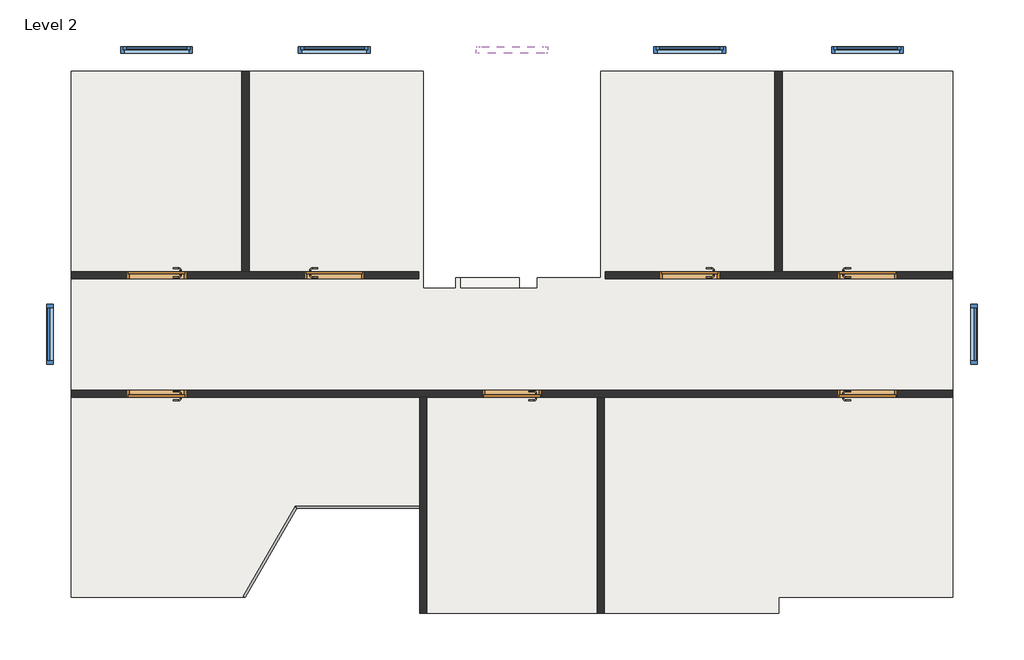
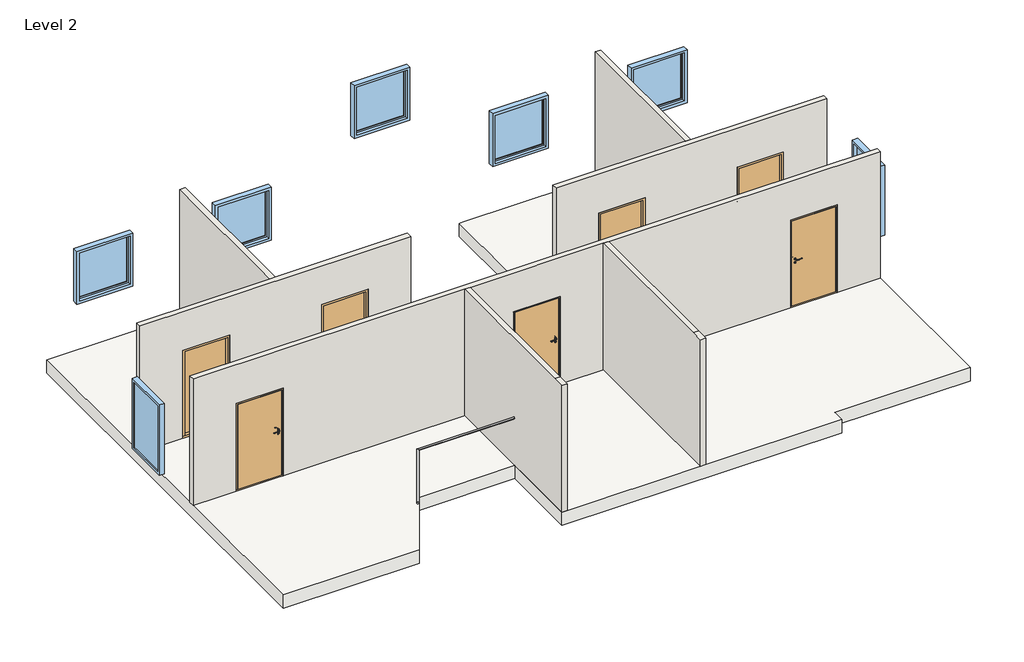
# One storey: 7 doors, 7 walls, 7 windows, 1 railing, 1 slab.
"""IFC4 building model written with IfcOpenShell, lengths in millimetres."""

import ifcopenshell
import ifcopenshell.guid

model = None  # the IFC model being written
_history = None  # IfcOwnerHistory: only IFC2X3 demands one
_inside = {}  # id of a spatial element -> (the spatial element, [elements in it])
_under = {}  # id of a project, library or spatial element -> (it, [spatial elements below it])
_declared = {}  # id of a project -> (the project, [libraries it declares])
_typed = {}  # id of a type object -> (the type object, [elements of that type])
_made_of = {}  # id of a material, layer set ... -> (it, [elements and type objects made of it])


def new_model(schema):
    """Start an empty IFC model of exactly this schema.

    Asked for "IFC4X3", IfcOpenShell would pick the latest addendum, in which some entities
    have other attributes; the version numbers below select the first issue.
    IFC2X3 requires an IfcOwnerHistory on every rooted entity: one is made here for all.
    """
    global model, _history
    if schema == "IFC4X3":
        model = ifcopenshell.file(schema_version=(4, 3, 0, 0))
    else:
        model = ifcopenshell.file(schema=schema)
    _inside.clear()
    _under.clear()
    _declared.clear()
    _typed.clear()
    _made_of.clear()
    _history = None
    if model.schema == "IFC2X3":
        org = make("IfcOrganization", Name="unknown")
        user = make(
            "IfcPersonAndOrganization",
            ThePerson=make("IfcPerson", FamilyName="unknown"),
            TheOrganization=org,
        )
        app = make(
            "IfcApplication",
            ApplicationDeveloper=org,
            Version="unknown",
            ApplicationFullName="unknown",
            ApplicationIdentifier="unknown",
        )
        _history = make(
            "IfcOwnerHistory",
            OwningUser=user,
            OwningApplication=app,
            ChangeAction="ADDED",
            CreationDate=0,
        )
    return model


def make(cls, **values):
    """One entity of the class cls with the attributes given. An attribute that is None is left unset."""
    return model.create_entity(
        cls, **{name: value for name, value in values.items() if value is not None}
    )


def rooted(cls, **values):
    """An entity with a GlobalId (a new one), such as an element, a storey or a relation."""
    return make(cls, GlobalId=ifcopenshell.guid.new(), OwnerHistory=_history, **values)


def si_unit(unit_type, name, prefix=None):
    """IfcSIUnit, for example si_unit("LENGTHUNIT", "METRE", prefix="MILLI")."""
    return make("IfcSIUnit", UnitType=unit_type, Prefix=prefix, Name=name)


def assignment(units):
    """IfcUnitAssignment: the units of a project."""
    return None if units is None else make("IfcUnitAssignment", Units=units)


def point(xyz):
    """IfcCartesianPoint."""
    return None if xyz is None else make("IfcCartesianPoint", Coordinates=xyz)


def direction(xyz):
    """IfcDirection."""
    return None if xyz is None else make("IfcDirection", DirectionRatios=xyz)


def frame(location, z_axis=None, x_axis=None):
    """IfcAxis2Placement3D, a coordinate frame: its origin and axes. An axis left out is left unset."""
    return make(
        "IfcAxis2Placement3D",
        Location=point(location),
        Axis=direction(z_axis),
        RefDirection=direction(x_axis),
    )


def frame_2d(location, x_axis=None):
    """IfcAxis2Placement2D, a coordinate frame in the plane: its origin and x axis."""
    return make(
        "IfcAxis2Placement2D", Location=point(location), RefDirection=direction(x_axis)
    )


def origin():
    """The frame at (0, 0, 0) with its axes left unset."""
    return frame((0.0, 0.0, 0.0))


def place(relative_to, where):
    """IfcLocalPlacement: puts the frame where relative to a parent placement (None: the world)."""
    return make(
        "IfcLocalPlacement", PlacementRelTo=relative_to, RelativePlacement=where
    )


def context(
    kind, dimensions, precision=None, world=None, true_north=None, identifier=None
):
    """IfcGeometricRepresentationContext, for example the 3D "Model" context."""
    return make(
        "IfcGeometricRepresentationContext",
        ContextIdentifier=identifier,
        ContextType=kind,
        CoordinateSpaceDimension=dimensions,
        Precision=precision,
        WorldCoordinateSystem=world,
        TrueNorth=true_north,
    )


def project(units=None, contexts=None):
    """IfcProject with its units and contexts."""
    return rooted(
        "IfcProject",
        Name="project",
        RepresentationContexts=contexts,
        UnitsInContext=assignment(units),
    )


def spatial(cls, under=None, at=None, **own):
    """A site, building, storey or space (cls), placed at a placement, below another one or the project."""
    s = rooted(cls, ObjectPlacement=at, **own)
    if under is not None:
        _under.setdefault(under.id(), (under, []))[1].append(s)
    return s


def polyline(points):
    """IfcPolyline through the points."""
    return make("IfcPolyline", Points=[point(p) for p in points])


def circle_curve(where, radius):
    """IfcCircle in the frame where."""
    return make("IfcCircle", Position=where, Radius=radius)


def ellipse_curve(where, semi_axis1, semi_axis2):
    """IfcEllipse in the frame where."""
    return make(
        "IfcEllipse", Position=where, SemiAxis1=semi_axis1, SemiAxis2=semi_axis2
    )


def trimmed(basis, trim1, trim2, sense, master):
    """IfcTrimmedCurve: the piece of a basis curve between two trims."""
    return make(
        "IfcTrimmedCurve",
        BasisCurve=basis,
        Trim1=trim1,
        Trim2=trim2,
        SenseAgreement=sense,
        MasterRepresentation=master,
    )


def segment(curve, same_sense, transition):
    """IfcCompositeCurveSegment."""
    return make(
        "IfcCompositeCurveSegment",
        Transition=transition,
        SameSense=same_sense,
        ParentCurve=curve,
    )


def composite_curve(segments, self_intersect=None):
    """IfcCompositeCurve: segments joined end to end."""
    return make("IfcCompositeCurve", Segments=segments, SelfIntersect=self_intersect)


def outline(outer, holes=None, kind="AREA"):
    """IfcArbitraryClosedProfileDef: a profile drawn as a closed curve; with holes, ...WithVoids."""
    if holes is None:
        return make("IfcArbitraryClosedProfileDef", ProfileType=kind, OuterCurve=outer)
    return make(
        "IfcArbitraryProfileDefWithVoids",
        ProfileType=kind,
        OuterCurve=outer,
        InnerCurves=holes,
    )


def extrude(swept, where, along, depth):
    """IfcExtrudedAreaSolid: the profile swept, set in the frame where, extruded along a direction by depth."""
    return make(
        "IfcExtrudedAreaSolid",
        SweptArea=swept,
        Position=where,
        ExtrudedDirection=direction(along),
        Depth=depth,
    )


def faces_of(points, faces, orient=None, outer=None):
    """IfcFace entities. A face is a list of loops; a loop is a list of indices into points, from 0.

    orient and outer hold one flag for each loop. By default every Orientation is true, the
    first loop of a face is its IfcFaceOuterBound and the others are IfcFaceBound.
    """
    made = []
    for i, loops in enumerate(faces):
        bounds = []
        for j, loop in enumerate(loops):
            is_outer = j == 0 if outer is None else outer[i][j]
            bounds.append(
                make(
                    "IfcFaceOuterBound" if is_outer else "IfcFaceBound",
                    Bound=make("IfcPolyLoop", Polygon=[points[k] for k in loop]),
                    Orientation=True if orient is None else orient[i][j],
                )
            )
        made.append(make("IfcFace", Bounds=bounds))
    return made


def faceted_brep(points, faces, orient=None, outer=None, voids=None):
    """IfcFacetedBrep: a solid bounded by flat faces; with voids (closed shells), ...WithVoids."""
    shared = [point(p) for p in points]
    hull = make("IfcClosedShell", CfsFaces=faces_of(shared, faces, orient, outer))
    if voids is None:
        return make("IfcFacetedBrep", Outer=hull)
    return make(
        "IfcFacetedBrepWithVoids",
        Outer=hull,
        Voids=[
            make(cls, CfsFaces=faces_of(shared, fs, o, b)) for cls, fs, o, b in voids
        ],
    )


def shape(context_of_items, identifier, shape_type, items):
    """IfcShapeRepresentation: the items that make up one representation, for example the "Body"."""
    return make(
        "IfcShapeRepresentation",
        ContextOfItems=context_of_items,
        RepresentationIdentifier=identifier,
        RepresentationType=shape_type,
        Items=items,
    )


def source(mapping_origin, context_of_items, identifier, shape_type, items):
    """IfcRepresentationMap: a shape defined once, which mapped items show again and again."""
    return make(
        "IfcRepresentationMap",
        MappingOrigin=mapping_origin,
        MappedRepresentation=shape(context_of_items, identifier, shape_type, items),
    )


def transform(
    local_origin,
    x_axis=None,
    y_axis=None,
    z_axis=None,
    scale=None,
    scale2=None,
    scale3=None,
    uniform=True,
):
    """IfcCartesianTransformationOperator3D, or its non-uniform kind. x_axis, y_axis, z_axis: its Axis1, 2, 3."""
    if uniform:
        return make(
            "IfcCartesianTransformationOperator3D",
            Axis1=direction(x_axis),
            Axis2=direction(y_axis),
            LocalOrigin=point(local_origin),
            Scale=scale,
            Axis3=direction(z_axis),
        )
    return make(
        "IfcCartesianTransformationOperator3DnonUniform",
        Axis1=direction(x_axis),
        Axis2=direction(y_axis),
        LocalOrigin=point(local_origin),
        Scale=scale,
        Axis3=direction(z_axis),
        Scale2=scale2,
        Scale3=scale3,
    )


def mapped(mapping_source, mapping_target):
    """IfcMappedItem: shows the shape of a source again, moved by a transform."""
    return make(
        "IfcMappedItem", MappingSource=mapping_source, MappingTarget=mapping_target
    )


def made_of(thing, what):
    """Note that an element or type object is made of a material, layer set ...; save() writes the relation."""
    if what is not None:
        _made_of.setdefault(what.id(), (what, []))[1].append(thing)
    return thing


def element(
    cls,
    number,
    at=None,
    inside=None,
    cuts=None,
    type_object=None,
    material=None,
    context=None,
    identifier="Body",
    shape_type=None,
    held_by="IfcProductDefinitionShape",
    body=None,
    shapes=None,
    **own,
):
    """One element of the class cls, such as IfcWall. Its Tag is "e" and its number.

    at: its placement. inside: the storey or other place that contains it. cuts: it is an
    opening in that element (IfcRelVoidsElement). A single representation is given by context,
    identifier, shape_type and body (its items); several are given by shapes. held_by: the class
    of the entity that holds the representations. save() writes the other relations.
    """
    e = rooted(cls, Tag="e%d" % number, ObjectPlacement=at, **own)
    if body is not None:
        shapes = [shape(context, identifier, shape_type, body)]
    if shapes is not None:
        e.Representation = make(held_by, Representations=shapes)
    if inside is not None:
        _inside.setdefault(inside.id(), (inside, []))[1].append(e)
    if cuts is not None:
        rooted(
            "IfcRelVoidsElement", RelatingBuildingElement=cuts, RelatedOpeningElement=e
        )
    if type_object is not None:
        _typed.setdefault(type_object.id(), (type_object, []))[1].append(e)
    return made_of(e, material)


def aggregate(whole, parts):
    """IfcRelAggregates: a whole, such as a stair, and the parts it consists of."""
    return rooted("IfcRelAggregates", RelatingObject=whole, RelatedObjects=parts)


def save(model, path):
    """Write the relations noted so far, then the file.

    IfcRelAggregates (storeys below a building ...), IfcRelContainedInSpatialStructure (elements
    in a storey), IfcRelDefinesByType, IfcRelAssociatesMaterial and IfcRelDeclares: one each for
    every whole, place, type object, material and project.
    """
    for whole, parts in _under.values():
        aggregate(whole, parts)
    for where, things in _inside.values():
        rooted(
            "IfcRelContainedInSpatialStructure",
            RelatedElements=things,
            RelatingStructure=where,
        )
    for kind, things in _typed.values():
        rooted("IfcRelDefinesByType", RelatedObjects=things, RelatingType=kind)
    for what, things in _made_of.values():
        rooted("IfcRelAssociatesMaterial", RelatedObjects=things, RelatingMaterial=what)
    for by, libraries in _declared.values():
        rooted("IfcRelDeclares", RelatingContext=by, RelatedDefinitions=libraries)
    model.write(path)


def plane_surface(at):
    """IfcPlane: the flat surface through the origin of the frame at, square to its z axis."""
    return make("IfcPlane", Position=at)


def cylinder_surface(at, radius):
    """IfcCylindricalSurface: all points at the distance radius from the z axis of the frame at."""
    return make("IfcCylindricalSurface", Position=at, Radius=radius)


def revolved_surface(curve, axis_point, axis_direction):
    """IfcSurfaceOfRevolution: the curve turned about the line through axis_point along axis_direction."""
    return make(
        "IfcSurfaceOfRevolution",
        SweptCurve=make("IfcArbitraryOpenProfileDef", ProfileType="CURVE", Curve=curve),
        AxisPosition=make("IfcAxis1Placement", Location=point(axis_point), Axis=direction(axis_direction)),
    )


def advanced_brep(points, edges, surfaces, faces):
    """IfcAdvancedBrep: a solid bounded by faces that lie on surfaces and meet in shared edges.

    An edge is (start, end): straight between two places in points (the first is 0);
    or (start, end, curve); or (start, end, curve, False) where it runs against its curve.
    A face is (place in surfaces, loops), or (place, loops, False) where it looks against
    its surface's normal. A loop lists edges by number (the first is 1), with a minus sign
    where the edge is run from its end to its start. The first loop is the outer one.
    """
    corners = [point(p) for p in points]
    vertices = [make("IfcVertexPoint", VertexGeometry=c) for c in corners]
    made = []
    for start, end, *more in edges:
        made.append(
            make(
                "IfcEdgeCurve",
                EdgeStart=vertices[start],
                EdgeEnd=vertices[end],
                EdgeGeometry=more[0] if more else make("IfcPolyline", Points=[corners[start], corners[end]]),
                SameSense=more[1] if len(more) > 1 else True,
            )
        )
    hull = []
    for where, loops, *sense in faces:
        bounds = []
        for j, loop in enumerate(loops):
            ring = [make("IfcOrientedEdge", EdgeElement=made[abs(k) - 1], Orientation=k > 0) for k in loop]
            bounds.append(
                make(
                    "IfcFaceOuterBound" if j == 0 else "IfcFaceBound",
                    Bound=make("IfcEdgeLoop", EdgeList=ring),
                    Orientation=True,
                )
            )
        hull.append(make("IfcAdvancedFace", Bounds=bounds, FaceSurface=surfaces[where], SameSense=sense[0] if sense else True))
    return make("IfcAdvancedBrep", Outer=make("IfcClosedShell", CfsFaces=hull))


def int_single_flush_10x20m_e84bf50b(model_context):
    return source(origin(), model_context, "Body", "SolidModel", [
        extrude(outline(composite_curve([segment(trimmed(circle_curve(frame_2d((1090.0, -406.0)), 20.0), [point((1070.0, -406.0))], [point((1110.0, -406.0))], False, "CARTESIAN"), True, "CONTINUOUS"), segment(trimmed(circle_curve(frame_2d((1090.0, -406.0)), 20.0), [point((1110.0, -406.0))], [point((1070.0, -406.0))], False, "CARTESIAN"), True, "CONTINUOUS")], self_intersect=False)), frame((0.0, 60.0, 0.0), z_axis=(0.0, 1.0, 0.0), x_axis=(0.0, 0.0, 1.0)), (0.0, 0.0, 1.0), 2.0),
        advanced_brep(
        [(-413.5, 62.0, 1090.0), (-398.5, 62.0, 1090.0), (-413.5, 84.5, 1090.0), (-398.5, 84.5, 1090.0), (-376.0, 107.0, 1090.0), (-376.0, 122.0, 1090.0), (-281.0, 122.0, 1090.0), (-281.0, 107.0, 1090.0)],
        [
            (0, 1, circle_curve(frame((-406.0, 62.0, 1090.0), z_axis=(0.0, -1.0, 0.0), x_axis=(1.0, 0.0, 0.0)), 7.5)),
            (1, 0, circle_curve(frame((-406.0, 62.0, 1090.0), z_axis=(0.0, -1.0, 0.0), x_axis=(1.0, 0.0, 0.0)), 7.5)),
            (0, 2),
            (2, 3, circle_curve(frame((-406.0, 84.5, 1090.0), z_axis=(0.0, -1.0, 0.0), x_axis=(1.0, 0.0, 0.0)), 7.5)),
            (3, 1),
            (3, 2, circle_curve(frame((-406.0, 84.5, 1090.0), z_axis=(0.0, -1.0, 0.0), x_axis=(1.0, 0.0, 0.0)), 7.5)),
            (4, 3, circle_curve(frame((-376.0, 84.5, 1090.0), z_axis=(0.0, 0.0, 1.0), x_axis=(-1.0, 0.0, 0.0)), 22.5)),
            (2, 5, circle_curve(frame((-376.0, 84.5, 1090.0), z_axis=(0.0, 0.0, -1.0), x_axis=(-1.0, 0.0, 0.0)), 37.5)),
            (5, 4, circle_curve(frame((-376.0, 114.5, 1090.0), z_axis=(-1.0, 0.0, 0.0), x_axis=(0.0, -1.0, 0.0)), 7.5)),
            (4, 5, circle_curve(frame((-376.0, 114.5, 1090.0), z_axis=(-1.0, 0.0, 0.0), x_axis=(0.0, -1.0, 0.0)), 7.5)),
            (5, 6),
            (6, 7, circle_curve(frame((-281.0, 114.5, 1090.0), z_axis=(-1.0, 0.0, 0.0), x_axis=(0.0, -1.0, 0.0)), 7.5)),
            (7, 4),
            (7, 6, circle_curve(frame((-281.0, 114.5, 1090.0), z_axis=(-1.0, 0.0, 0.0), x_axis=(0.0, -1.0, 0.0)), 7.5)),
        ],
        [
            plane_surface(frame((-406.0, 62.0, 1090.0), z_axis=(0.0, -1.0, 0.0), x_axis=(0.0, 0.0, -1.0))),
            cylinder_surface(frame((-406.0, 62.0, 1090.0), z_axis=(0.0, -1.0, 0.0), x_axis=(1.0, 0.0, 0.0)), 7.5),
            revolved_surface(trimmed(ellipse_curve(frame((-406.0, 84.5, 1090.0), z_axis=(0.0, -1.0, 0.0), x_axis=(1.0, 0.0, 0.0)), 7.5, 7.5), [point((-413.5, 84.5, 1090.0))], [point((-398.5, 84.5, 1090.0))], True, "CARTESIAN"), (-376.0, 84.5, 1090.0), (0.0, 0.0, -1.0)),
            revolved_surface(trimmed(ellipse_curve(frame((-406.0, 84.5, 1090.0), z_axis=(0.0, -1.0, 0.0), x_axis=(1.0, 0.0, 0.0)), 7.5, 7.5), [point((-398.5, 84.5, 1090.0))], [point((-413.5, 84.5, 1090.0))], True, "CARTESIAN"), (-376.0, 84.5, 1090.0), (0.0, 0.0, -1.0)),
            cylinder_surface(frame((-376.0, 114.5, 1090.0), z_axis=(-1.0, 0.0, 0.0), x_axis=(0.0, -1.0, 0.0)), 7.5),
            plane_surface(frame((-281.0, 114.5, 1090.0), z_axis=(1.0, 0.0, 0.0), x_axis=(0.0, 0.0, -1.0))),
        ],
        [
            (0, [[1, 2]]),
            (1, [[-1, 3, 4, 5]]),
            (1, [[-2, -5, 6, -3]]),
            (2, [[7, -4, 8, 9]]),
            (3, [[-8, -6, -7, 10]]),
            (4, [[-9, 11, 12, 13]]),
            (4, [[-10, -13, 14, -11]]),
            (5, [[-14, -12]]),
        ],
    ),
        extrude(outline(composite_curve([segment(trimmed(circle_curve(frame_2d((1010.0, -406.0)), 20.0), [point((990.0, -406.0))], [point((1030.0, -406.0))], False, "CARTESIAN"), True, "CONTINUOUS"), segment(trimmed(circle_curve(frame_2d((1010.0, -406.0)), 20.0), [point((1030.0, -406.0))], [point((990.0, -406.0))], False, "CARTESIAN"), True, "CONTINUOUS")], self_intersect=False), holes=[composite_curve([segment(trimmed(circle_curve(frame_2d((1015.0, -406.0)), 3.0), [point((1012.4019238, -407.5))], [point((1012.4019238, -404.5))], True, "CARTESIAN"), True, "CONTINUOUS"), segment(polyline([(1012.4019238, -404.5), (1000.0, -404.5), (1000.0, -407.5), (1012.4019238, -407.5)]), True, "CONTINUOUS")], self_intersect=False)]), frame((0.0, 60.0, 0.0), z_axis=(0.0, 1.0, 0.0), x_axis=(0.0, 0.0, 1.0)), (0.0, 0.0, 1.0), 2.0),
        extrude(outline(composite_curve([segment(trimmed(circle_curve(frame_2d((1090.0, -406.0)), 20.0), [point((1070.0, -406.0))], [point((1110.0, -406.0))], False, "CARTESIAN"), True, "CONTINUOUS"), segment(trimmed(circle_curve(frame_2d((1090.0, -406.0)), 20.0), [point((1110.0, -406.0))], [point((1070.0, -406.0))], False, "CARTESIAN"), True, "CONTINUOUS")], self_intersect=False)), frame((0.0, 18.0, 0.0), z_axis=(0.0, 1.0, 0.0), x_axis=(0.0, 0.0, 1.0)), (0.0, 0.0, 1.0), 2.0),
        advanced_brep(
        [(-413.5, 18.0, 1090.0), (-398.5, 18.0, 1090.0), (-398.5, -4.5, 1090.0), (-413.5, -4.5, 1090.0), (-376.0, -27.0, 1090.0), (-376.0, -42.0, 1090.0), (-281.0, -27.0, 1090.0), (-281.0, -42.0, 1090.0)],
        [
            (0, 1, circle_curve(frame((-406.0, 18.0, 1090.0), z_axis=(0.0, 1.0, 0.0), x_axis=(1.0, 0.0, 0.0)), 7.5)),
            (1, 0, circle_curve(frame((-406.0, 18.0, 1090.0), z_axis=(0.0, 1.0, 0.0), x_axis=(1.0, 0.0, 0.0)), 7.5)),
            (1, 2),
            (2, 3, circle_curve(frame((-406.0, -4.5, 1090.0), z_axis=(0.0, 1.0, 0.0), x_axis=(1.0, 0.0, 0.0)), 7.5)),
            (3, 0),
            (3, 2, circle_curve(frame((-406.0, -4.5, 1090.0), z_axis=(0.0, 1.0, 0.0), x_axis=(1.0, 0.0, 0.0)), 7.5)),
            (4, 5, circle_curve(frame((-376.0, -34.5, 1090.0), z_axis=(-1.0, 0.0, 0.0), x_axis=(0.0, 1.0, 0.0)), 7.5)),
            (5, 3, circle_curve(frame((-376.0, -4.5, 1090.0), z_axis=(0.0, 0.0, -1.0), x_axis=(-1.0, 0.0, 0.0)), 37.5)),
            (2, 4, circle_curve(frame((-376.0, -4.5, 1090.0), z_axis=(0.0, 0.0, 1.0), x_axis=(-1.0, 0.0, 0.0)), 22.5)),
            (5, 4, circle_curve(frame((-376.0, -34.5, 1090.0), z_axis=(-1.0, 0.0, 0.0), x_axis=(0.0, 1.0, 0.0)), 7.5)),
            (4, 6),
            (6, 7, circle_curve(frame((-281.0, -34.5, 1090.0), z_axis=(-1.0, 0.0, 0.0), x_axis=(0.0, 1.0, 0.0)), 7.5)),
            (7, 5),
            (7, 6, circle_curve(frame((-281.0, -34.5, 1090.0), z_axis=(-1.0, 0.0, 0.0), x_axis=(0.0, 1.0, 0.0)), 7.5)),
        ],
        [
            plane_surface(frame((-406.0, 18.0, 1090.0), z_axis=(0.0, 1.0, 0.0), x_axis=(0.0, 0.0, -1.0))),
            cylinder_surface(frame((-406.0, 18.0, 1090.0), z_axis=(0.0, 1.0, 0.0), x_axis=(1.0, 0.0, 0.0)), 7.5),
            revolved_surface(trimmed(ellipse_curve(frame((-406.0, -4.5, 1090.0), z_axis=(0.0, -1.0, 0.0), x_axis=(1.0, 0.0, 0.0)), 7.5, 7.5), [point((-413.5, -4.5, 1090.0))], [point((-398.5, -4.5, 1090.0))], True, "CARTESIAN"), (-376.0, -4.5, 1090.0), (0.0, 0.0, -1.0)),
            revolved_surface(trimmed(ellipse_curve(frame((-406.0, -4.5, 1090.0), z_axis=(0.0, -1.0, 0.0), x_axis=(1.0, 0.0, 0.0)), 7.5, 7.5), [point((-398.5, -4.5, 1090.0))], [point((-413.5, -4.5, 1090.0))], True, "CARTESIAN"), (-376.0, -4.5, 1090.0), (0.0, 0.0, -1.0)),
            cylinder_surface(frame((-376.0, -34.5, 1090.0), z_axis=(-1.0, 0.0, 0.0), x_axis=(0.0, 1.0, 0.0)), 7.5),
            plane_surface(frame((-281.0, -34.5, 1090.0), z_axis=(1.0, 0.0, 0.0), x_axis=(0.0, 0.0, -1.0))),
        ],
        [
            (0, [[1, 2]]),
            (1, [[3, 4, 5, -2]]),
            (1, [[-5, 6, -3, -1]]),
            (2, [[7, 8, -4, 9]]),
            (3, [[10, -9, -6, -8]]),
            (4, [[11, 12, 13, -7]]),
            (4, [[-13, 14, -11, -10]]),
            (5, [[-12, -14]]),
        ],
    ),
        extrude(outline(composite_curve([segment(trimmed(circle_curve(frame_2d((1010.0, -406.0)), 20.0), [point((990.0, -406.0))], [point((1030.0, -406.0))], False, "CARTESIAN"), True, "CONTINUOUS"), segment(trimmed(circle_curve(frame_2d((1010.0, -406.0)), 20.0), [point((1030.0, -406.0))], [point((990.0, -406.0))], False, "CARTESIAN"), True, "CONTINUOUS")], self_intersect=False), holes=[composite_curve([segment(trimmed(circle_curve(frame_2d((1015.0, -406.0)), 3.0), [point((1012.4019238, -407.5))], [point((1012.4019238, -404.5))], True, "CARTESIAN"), True, "CONTINUOUS"), segment(polyline([(1012.4019238, -404.5), (1000.0, -404.5), (1000.0, -407.5), (1012.4019238, -407.5)]), True, "CONTINUOUS")], self_intersect=False)]), frame((0.0, 18.0, 0.0), z_axis=(0.0, 1.0, 0.0), x_axis=(0.0, 0.0, 1.0)), (0.0, 0.0, 1.0), 2.0),
        extrude(outline(polyline([(476.0, 20.0), (-476.0, 20.0), (-476.0, 60.0), (476.0, 60.0), (476.0, 20.0)])), frame((0.0, 0.0, 30.0), z_axis=(0.0, 0.0, 1.0), x_axis=(1.0, 0.0, 0.0)), (0.0, 0.0, 1.0), 1952.0),
        extrude(outline(polyline([(20.0, 42.0), (20.0, 30.0), (60.0, 30.0), (60.0, 0.0), (-60.0, 0.0), (-60.0, 42.0), (20.0, 42.0)])), frame((-506.0, 0.0, 0.0), z_axis=(1.0, 0.0, 0.0), x_axis=(0.0, 1.0, 0.0)), (0.0, 0.0, 1.0), 1012.0),
        faceted_brep([(-476.0, 20.0, 1982.0), (476.0, 20.0, 1982.0), (476.0, 20.0, 42.0), (464.0, 20.0, 42.0), (464.0, 20.0, 1970.0), (-464.0, 20.0, 1970.0), (-464.0, 20.0, 42.0), (-476.0, 20.0, 42.0), (-476.0, 60.0, 1982.0), (-476.0, 20.0, 30.0), (-476.0, 60.0, 30.0), (-506.0, 20.0, 42.0), (-506.0, 20.0, 30.0), (506.0, 20.0, 42.0), (476.0, 20.0, 30.0), (506.0, 20.0, 30.0), (-506.0, 60.0, 30.0), (476.0, 60.0, 30.0), (506.0, 60.0, 30.0), (-506.0, 60.0, 2012.0), (506.0, 60.0, 2012.0), (476.0, 60.0, 1982.0), (-464.0, -60.0, 42.0), (-506.0, -60.0, 42.0), (506.0, -60.0, 42.0), (464.0, -60.0, 42.0), (464.0, -60.0, 1970.0), (-464.0, -60.0, 1970.0), (506.0, -60.0, 2012.0), (-506.0, -60.0, 2012.0)], [[[0, 1, 2, 3, 4, 5, 6, 7]], [[8, 0, 7, 9, 10]], [[7, 11, 12, 9]], [[13, 2, 14, 15]], [[9, 12, 16, 10]], [[15, 14, 17, 18]], [[19, 20, 18, 17, 21, 8, 10, 16]], [[1, 21, 17, 14, 2]], [[11, 7, 6, 22, 23]], [[2, 13, 24, 25, 3]], [[26, 4, 3, 25]], [[5, 27, 22, 6]], [[27, 26, 25, 24, 28, 29, 23, 22]], [[20, 28, 24, 13, 15, 18]], [[29, 19, 16, 12, 11, 23]], [[0, 8, 21, 1]], [[5, 4, 26, 27]], [[29, 28, 20, 19]]]),
    ])


def int_single_flush_10x20m_68751a9d(model_context):
    return source(origin(), model_context, "Body", "SolidModel", [
        extrude(outline(composite_curve([segment(trimmed(circle_curve(frame_2d((1090.0, -406.0)), 20.0), [point((1070.0, -406.0))], [point((1110.0, -406.0))], False, "CARTESIAN"), True, "CONTINUOUS"), segment(trimmed(circle_curve(frame_2d((1090.0, -406.0)), 20.0), [point((1110.0, -406.0))], [point((1070.0, -406.0))], False, "CARTESIAN"), True, "CONTINUOUS")], self_intersect=False)), frame((0.0, -62.0, 0.0), z_axis=(0.0, 1.0, 0.0), x_axis=(0.0, 0.0, 1.0)), (0.0, 0.0, 1.0), 2.0),
        advanced_brep(
        [(-413.5, -62.0, 1090.0), (-398.5, -62.0, 1090.0), (-398.5, -84.5, 1090.0), (-413.5, -84.5, 1090.0), (-376.0, -107.0, 1090.0), (-376.0, -122.0, 1090.0), (-281.0, -107.0, 1090.0), (-281.0, -122.0, 1090.0)],
        [
            (0, 1, circle_curve(frame((-406.0, -62.0, 1090.0), z_axis=(0.0, 1.0, 0.0), x_axis=(1.0, 0.0, 0.0)), 7.5)),
            (1, 0, circle_curve(frame((-406.0, -62.0, 1090.0), z_axis=(0.0, 1.0, 0.0), x_axis=(1.0, 0.0, 0.0)), 7.5)),
            (1, 2),
            (2, 3, circle_curve(frame((-406.0, -84.5, 1090.0), z_axis=(0.0, 1.0, 0.0), x_axis=(1.0, 0.0, 0.0)), 7.5)),
            (3, 0),
            (3, 2, circle_curve(frame((-406.0, -84.5, 1090.0), z_axis=(0.0, 1.0, 0.0), x_axis=(1.0, 0.0, 0.0)), 7.5)),
            (4, 5, circle_curve(frame((-376.0, -114.5, 1090.0), z_axis=(-1.0, 0.0, 0.0), x_axis=(0.0, 1.0, 0.0)), 7.5)),
            (5, 3, circle_curve(frame((-376.0, -84.5, 1090.0), z_axis=(0.0, 0.0, -1.0), x_axis=(-1.0, 0.0, 0.0)), 37.5)),
            (2, 4, circle_curve(frame((-376.0, -84.5, 1090.0), z_axis=(0.0, 0.0, 1.0), x_axis=(-1.0, 0.0, 0.0)), 22.5)),
            (5, 4, circle_curve(frame((-376.0, -114.5, 1090.0), z_axis=(-1.0, 0.0, 0.0), x_axis=(0.0, 1.0, 0.0)), 7.5)),
            (4, 6),
            (6, 7, circle_curve(frame((-281.0, -114.5, 1090.0), z_axis=(-1.0, 0.0, 0.0), x_axis=(0.0, 1.0, 0.0)), 7.5)),
            (7, 5),
            (7, 6, circle_curve(frame((-281.0, -114.5, 1090.0), z_axis=(-1.0, 0.0, 0.0), x_axis=(0.0, 1.0, 0.0)), 7.5)),
        ],
        [
            plane_surface(frame((-406.0, -62.0, 1090.0), z_axis=(0.0, 1.0, 0.0), x_axis=(0.0, 0.0, -1.0))),
            cylinder_surface(frame((-406.0, -62.0, 1090.0), z_axis=(0.0, 1.0, 0.0), x_axis=(1.0, 0.0, 0.0)), 7.5),
            revolved_surface(trimmed(ellipse_curve(frame((-406.0, -84.5, 1090.0), z_axis=(0.0, -1.0, 0.0), x_axis=(1.0, 0.0, 0.0)), 7.5, 7.5), [point((-413.5, -84.5, 1090.0))], [point((-398.5, -84.5, 1090.0))], True, "CARTESIAN"), (-376.0, -84.5, 1090.0), (0.0, 0.0, -1.0)),
            revolved_surface(trimmed(ellipse_curve(frame((-406.0, -84.5, 1090.0), z_axis=(0.0, -1.0, 0.0), x_axis=(1.0, 0.0, 0.0)), 7.5, 7.5), [point((-398.5, -84.5, 1090.0))], [point((-413.5, -84.5, 1090.0))], True, "CARTESIAN"), (-376.0, -84.5, 1090.0), (0.0, 0.0, -1.0)),
            cylinder_surface(frame((-376.0, -114.5, 1090.0), z_axis=(-1.0, 0.0, 0.0), x_axis=(0.0, 1.0, 0.0)), 7.5),
            plane_surface(frame((-281.0, -114.5, 1090.0), z_axis=(1.0, 0.0, 0.0), x_axis=(0.0, 0.0, -1.0))),
        ],
        [
            (0, [[1, 2]]),
            (1, [[3, 4, 5, -2]]),
            (1, [[-5, 6, -3, -1]]),
            (2, [[7, 8, -4, 9]]),
            (3, [[10, -9, -6, -8]]),
            (4, [[11, 12, 13, -7]]),
            (4, [[-13, 14, -11, -10]]),
            (5, [[-12, -14]]),
        ],
    ),
        extrude(outline(composite_curve([segment(trimmed(circle_curve(frame_2d((1010.0, -406.0)), 20.0), [point((990.0, -406.0))], [point((1030.0, -406.0))], False, "CARTESIAN"), True, "CONTINUOUS"), segment(trimmed(circle_curve(frame_2d((1010.0, -406.0)), 20.0), [point((1030.0, -406.0))], [point((990.0, -406.0))], False, "CARTESIAN"), True, "CONTINUOUS")], self_intersect=False), holes=[composite_curve([segment(trimmed(circle_curve(frame_2d((1015.0, -406.0)), 3.0), [point((1012.4019238, -407.5))], [point((1012.4019238, -404.5))], True, "CARTESIAN"), True, "CONTINUOUS"), segment(polyline([(1012.4019238, -404.5), (1000.0, -404.5), (1000.0, -407.5), (1012.4019238, -407.5)]), True, "CONTINUOUS")], self_intersect=False)]), frame((0.0, -62.0, 0.0), z_axis=(0.0, 1.0, 0.0), x_axis=(0.0, 0.0, 1.0)), (0.0, 0.0, 1.0), 2.0),
        extrude(outline(composite_curve([segment(trimmed(circle_curve(frame_2d((1090.0, -406.0)), 20.0), [point((1070.0, -406.0))], [point((1110.0, -406.0))], False, "CARTESIAN"), True, "CONTINUOUS"), segment(trimmed(circle_curve(frame_2d((1090.0, -406.0)), 20.0), [point((1110.0, -406.0))], [point((1070.0, -406.0))], False, "CARTESIAN"), True, "CONTINUOUS")], self_intersect=False)), frame((0.0, -20.0, 0.0), z_axis=(0.0, 1.0, 0.0), x_axis=(0.0, 0.0, 1.0)), (0.0, 0.0, 1.0), 2.0),
        advanced_brep(
        [(-413.5, -18.0, 1090.0), (-398.5, -18.0, 1090.0), (-413.5, 4.5, 1090.0), (-398.5, 4.5, 1090.0), (-376.0, 27.0, 1090.0), (-376.0, 42.0, 1090.0), (-281.0, 42.0, 1090.0), (-281.0, 27.0, 1090.0)],
        [
            (0, 1, circle_curve(frame((-406.0, -18.0, 1090.0), z_axis=(0.0, -1.0, 0.0), x_axis=(1.0, 0.0, 0.0)), 7.5)),
            (1, 0, circle_curve(frame((-406.0, -18.0, 1090.0), z_axis=(0.0, -1.0, 0.0), x_axis=(1.0, 0.0, 0.0)), 7.5)),
            (0, 2),
            (2, 3, circle_curve(frame((-406.0, 4.5, 1090.0), z_axis=(0.0, -1.0, 0.0), x_axis=(1.0, 0.0, 0.0)), 7.5)),
            (3, 1),
            (3, 2, circle_curve(frame((-406.0, 4.5, 1090.0), z_axis=(0.0, -1.0, 0.0), x_axis=(1.0, 0.0, 0.0)), 7.5)),
            (4, 3, circle_curve(frame((-376.0, 4.5, 1090.0), z_axis=(0.0, 0.0, 1.0), x_axis=(-1.0, 0.0, 0.0)), 22.5)),
            (2, 5, circle_curve(frame((-376.0, 4.5, 1090.0), z_axis=(0.0, 0.0, -1.0), x_axis=(-1.0, 0.0, 0.0)), 37.5)),
            (5, 4, circle_curve(frame((-376.0, 34.5, 1090.0), z_axis=(-1.0, 0.0, 0.0), x_axis=(0.0, -1.0, 0.0)), 7.5)),
            (4, 5, circle_curve(frame((-376.0, 34.5, 1090.0), z_axis=(-1.0, 0.0, 0.0), x_axis=(0.0, -1.0, 0.0)), 7.5)),
            (5, 6),
            (6, 7, circle_curve(frame((-281.0, 34.5, 1090.0), z_axis=(-1.0, 0.0, 0.0), x_axis=(0.0, -1.0, 0.0)), 7.5)),
            (7, 4),
            (7, 6, circle_curve(frame((-281.0, 34.5, 1090.0), z_axis=(-1.0, 0.0, 0.0), x_axis=(0.0, -1.0, 0.0)), 7.5)),
        ],
        [
            plane_surface(frame((-406.0, -18.0, 1090.0), z_axis=(0.0, -1.0, 0.0), x_axis=(0.0, 0.0, -1.0))),
            cylinder_surface(frame((-406.0, -18.0, 1090.0), z_axis=(0.0, -1.0, 0.0), x_axis=(1.0, 0.0, 0.0)), 7.5),
            revolved_surface(trimmed(ellipse_curve(frame((-406.0, 4.5, 1090.0), z_axis=(0.0, -1.0, 0.0), x_axis=(1.0, 0.0, 0.0)), 7.5, 7.5), [point((-413.5, 4.5, 1090.0))], [point((-398.5, 4.5, 1090.0))], True, "CARTESIAN"), (-376.0, 4.5, 1090.0), (0.0, 0.0, -1.0)),
            revolved_surface(trimmed(ellipse_curve(frame((-406.0, 4.5, 1090.0), z_axis=(0.0, -1.0, 0.0), x_axis=(1.0, 0.0, 0.0)), 7.5, 7.5), [point((-398.5, 4.5, 1090.0))], [point((-413.5, 4.5, 1090.0))], True, "CARTESIAN"), (-376.0, 4.5, 1090.0), (0.0, 0.0, -1.0)),
            cylinder_surface(frame((-376.0, 34.5, 1090.0), z_axis=(-1.0, 0.0, 0.0), x_axis=(0.0, -1.0, 0.0)), 7.5),
            plane_surface(frame((-281.0, 34.5, 1090.0), z_axis=(1.0, 0.0, 0.0), x_axis=(0.0, 0.0, -1.0))),
        ],
        [
            (0, [[1, 2]]),
            (1, [[-1, 3, 4, 5]]),
            (1, [[-2, -5, 6, -3]]),
            (2, [[7, -4, 8, 9]]),
            (3, [[-8, -6, -7, 10]]),
            (4, [[-9, 11, 12, 13]]),
            (4, [[-10, -13, 14, -11]]),
            (5, [[-14, -12]]),
        ],
    ),
        extrude(outline(composite_curve([segment(trimmed(circle_curve(frame_2d((1010.0, -406.0)), 20.0), [point((990.0, -406.0))], [point((1030.0, -406.0))], False, "CARTESIAN"), True, "CONTINUOUS"), segment(trimmed(circle_curve(frame_2d((1010.0, -406.0)), 20.0), [point((1030.0, -406.0))], [point((990.0, -406.0))], False, "CARTESIAN"), True, "CONTINUOUS")], self_intersect=False), holes=[composite_curve([segment(trimmed(circle_curve(frame_2d((1015.0, -406.0)), 3.0), [point((1012.4019238, -407.5))], [point((1012.4019238, -404.5))], True, "CARTESIAN"), True, "CONTINUOUS"), segment(polyline([(1012.4019238, -404.5), (1000.0, -404.5), (1000.0, -407.5), (1012.4019238, -407.5)]), True, "CONTINUOUS")], self_intersect=False)]), frame((0.0, -20.0, 0.0), z_axis=(0.0, 1.0, 0.0), x_axis=(0.0, 0.0, 1.0)), (0.0, 0.0, 1.0), 2.0),
        extrude(outline(polyline([(476.0, -20.0), (476.0, -60.0), (-476.0, -60.0), (-476.0, -20.0), (476.0, -20.0)])), frame((0.0, 0.0, 30.0), z_axis=(0.0, 0.0, 1.0), x_axis=(1.0, 0.0, 0.0)), (0.0, 0.0, 1.0), 1952.0),
        extrude(outline(polyline([(-20.0, 42.0), (60.0, 42.0), (60.0, 0.0), (-60.0, 0.0), (-60.0, 30.0), (-20.0, 30.0), (-20.0, 42.0)])), frame((-506.0, 0.0, 0.0), z_axis=(1.0, 0.0, 0.0), x_axis=(0.0, 1.0, 0.0)), (0.0, 0.0, 1.0), 1012.0),
        faceted_brep([(-476.0, -20.0, 1982.0), (-476.0, -20.0, 42.0), (-464.0, -20.0, 42.0), (-464.0, -20.0, 1970.0), (464.0, -20.0, 1970.0), (464.0, -20.0, 42.0), (476.0, -20.0, 42.0), (476.0, -20.0, 1982.0), (-476.0, -60.0, 1982.0), (-476.0, -60.0, 30.0), (-476.0, -20.0, 30.0), (-506.0, -20.0, 30.0), (-506.0, -20.0, 42.0), (506.0, -20.0, 42.0), (506.0, -20.0, 30.0), (476.0, -20.0, 30.0), (-506.0, -60.0, 30.0), (506.0, -60.0, 30.0), (476.0, -60.0, 30.0), (-506.0, -60.0, 2012.0), (476.0, -60.0, 1982.0), (506.0, -60.0, 2012.0), (464.0, 60.0, 42.0), (506.0, 60.0, 42.0), (-506.0, 60.0, 42.0), (-464.0, 60.0, 42.0), (464.0, 60.0, 1970.0), (-464.0, 60.0, 1970.0), (-506.0, 60.0, 2012.0), (506.0, 60.0, 2012.0)], [[[0, 1, 2, 3, 4, 5, 6, 7]], [[8, 9, 10, 1, 0]], [[1, 10, 11, 12]], [[13, 14, 15, 6]], [[10, 9, 16, 11]], [[14, 17, 18, 15]], [[19, 16, 9, 8, 20, 18, 17, 21]], [[7, 6, 15, 18, 20]], [[6, 5, 22, 23, 13]], [[12, 24, 25, 2, 1]], [[26, 22, 5, 4]], [[3, 2, 25, 27]], [[27, 25, 24, 28, 29, 23, 22, 26]], [[21, 17, 14, 13, 23, 29]], [[28, 24, 12, 11, 16, 19]], [[0, 7, 20, 8]], [[3, 27, 26, 4]], [[28, 19, 21, 29]]]),
    ])


def sketch_1100mm_c51240ad(model_context):
    return source(origin(), model_context, "Body", "AdvancedBrep", [
        advanced_brep(
        [(3000.0, 60.0, 4280.0), (2965.3589838, 80.0, 4280.0), (3842.931393, 1600.0, 4280.0), (3866.0254038, 1560.0, 4280.0), (5940.0, 1560.0, 4280.0), (5940.0, 1600.0, 4280.0)],
        [
            (0, 1, circle_curve(frame((2982.6794919, 70.0, 4280.0), z_axis=(-0.5000000000000013, -0.8660254037844379, 0.0), x_axis=(-0.8660254037844379, 0.5000000000000013, 0.0)), 20.0)),
            (1, 0, circle_curve(frame((2982.6794919, 70.0, 4280.0), z_axis=(-0.5000000000000013, -0.8660254037844379, 0.0), x_axis=(-0.8660254037844379, 0.5000000000000013, 0.0)), 20.0)),
            (1, 2),
            (2, 3, ellipse_curve(frame((3854.4783984, 1580.0, 4280.0), z_axis=(-0.8660254037844398, -0.49999999999999795, 0.0), x_axis=(0.4999999999999979, -0.8660254037844398, 0.0)), 23.0940108, 20.0)),
            (3, 0),
            (3, 2, ellipse_curve(frame((3854.4783984, 1580.0, 4280.0), z_axis=(-0.8660254037844398, -0.49999999999999795, 0.0), x_axis=(0.4999999999999979, -0.8660254037844398, 0.0)), 23.0940108, 20.0)),
            (4, 5, circle_curve(frame((5940.0, 1580.0, 4280.0), z_axis=(1.0, 0.0, 0.0), x_axis=(0.0, 1.0, 0.0)), 20.0)),
            (5, 4, circle_curve(frame((5940.0, 1580.0, 4280.0), z_axis=(1.0, 0.0, 0.0), x_axis=(0.0, 1.0, 0.0)), 20.0)),
            (2, 5),
            (4, 3),
        ],
        [
            plane_surface(frame((2982.6794919, 70.0, 4300.0), z_axis=(-0.5000000000000014, -0.8660254037844379, 0.0), x_axis=(0.8660254037844379, -0.5000000000000014, 0.0))),
            cylinder_surface(frame((2982.6794919, 70.0, 4280.0), z_axis=(-0.5000000000000013, -0.8660254037844379, 0.0), x_axis=(-0.8660254037844379, 0.5000000000000013, 0.0)), 20.0),
            plane_surface(frame((5940.0, 1580.0, 4300.0), z_axis=(1.0, 0.0, 0.0), x_axis=(0.0, 1.0, 0.0))),
            cylinder_surface(frame((3854.4783984, 1580.0, 4280.0), z_axis=(-1.0, 0.0, 0.0), x_axis=(0.0, 1.0, 0.0)), 20.0),
        ],
        [
            (0, [[1, 2]]),
            (1, [[-2, 3, 4, 5]]),
            (1, [[-1, -5, 6, -3]]),
            (2, [[7, 8]]),
            (3, [[-4, 9, -7, 10]]),
            (3, [[-6, -10, -8, -9]]),
        ],
    ),
    ])


def fixed_10x16m_885135a8(model_context):
    return source(origin(), model_context, "Body", "SweptSolid", [
        extrude(outline(polyline([(2412.0, 506.0), (2412.0, -506.0), (800.0, -506.0), (800.0, 506.0), (2412.0, 506.0)]), holes=[polyline([(857.0, 449.0), (857.0, -449.0), (2355.0, -449.0), (2355.0, 449.0), (857.0, 449.0)])]), frame((0.0, 69.0, 0.0), z_axis=(0.0, 1.0, 0.0), x_axis=(0.0, 0.0, 1.0)), (0.0, 0.0, 1.0), 115.0),
        extrude(outline(polyline([(-449.0, 162.0), (449.0, 162.0), (449.0, 134.0), (-449.0, 134.0), (-449.0, 162.0)])), frame((0.0, 0.0, 857.0), z_axis=(0.0, 0.0, 1.0), x_axis=(1.0, 0.0, 0.0)), (0.0, 0.0, 1.0), 1498.0),
    ])


def single_light_12x12m_8659da90(model_context):
    return source(origin(), model_context, "Body", "SolidModel", [
        extrude(outline(polyline([(1970.0, -564.0), (842.0, -564.0), (842.0, 564.0), (1970.0, 564.0), (1970.0, -564.0)]), holes=[polyline([(1920.0, 514.0), (892.0, 514.0), (892.0, -514.0), (1920.0, -514.0), (1920.0, 514.0)])]), frame((0.0, 134.0, 0.0), z_axis=(0.0, 1.0, 0.0), x_axis=(0.0, 0.0, 1.0)), (0.0, 0.0, 1.0), 50.0),
        faceted_brep([(-606.0, 69.0, 800.0), (-606.0, 184.0, 800.0), (606.0, 184.0, 800.0), (606.0, 69.0, 800.0), (606.0, 184.0, 2012.0), (606.0, 69.0, 2012.0), (-606.0, 184.0, 2012.0), (564.0, 184.0, 1970.0), (-564.0, 184.0, 1970.0), (-564.0, 184.0, 842.0), (564.0, 184.0, 842.0), (-606.0, 69.0, 2012.0), (549.0, 69.0, 857.0), (-549.0, 69.0, 857.0), (-549.0, 69.0, 1955.0), (549.0, 69.0, 1955.0), (-549.0, 134.0, 857.0), (549.0, 134.0, 857.0), (549.0, 134.0, 1955.0), (564.0, 134.0, 842.0), (-564.0, 134.0, 842.0), (-564.0, 134.0, 1970.0), (564.0, 134.0, 1970.0), (-549.0, 134.0, 1955.0)], [[[0, 1, 2, 3]], [[3, 2, 4, 5]], [[2, 1, 6, 4], [7, 8, 9, 10]], [[5, 11, 0, 3], [12, 13, 14, 15]], [[16, 13, 12, 17]], [[17, 12, 15, 18]], [[19, 20, 21, 22], [18, 23, 16, 17]], [[9, 20, 19, 10]], [[10, 19, 22, 7]], [[11, 6, 1, 0]], [[23, 14, 13, 16]], [[8, 21, 20, 9]], [[5, 4, 6, 11]], [[18, 15, 14, 23]], [[7, 22, 21, 8]]]),
        extrude(outline(polyline([(-514.0, 170.0), (514.0, 170.0), (514.0, 148.0), (-514.0, 148.0), (-514.0, 170.0)])), frame((0.0, 0.0, 892.0), z_axis=(0.0, 0.0, 1.0), x_axis=(1.0, 0.0, 0.0)), (0.0, 0.0, 1.0), 1028.0),
    ])


model = new_model("IFC4")

# Units and contexts
model_context = context("Model", 3, world=origin())
ifc_project = project(units=[si_unit("LENGTHUNIT", "METRE", prefix="MILLI")], contexts=[model_context])

# Site, building, storey
site = spatial("IfcSite", under=ifc_project)
building = spatial("IfcBuilding", under=site)
storey = spatial("IfcBuildingStorey", under=building, Name="Level 2", Elevation=3200.0)

# Doors
placement = place(None, origin())
int_single_flush_10x20m_shape = int_single_flush_10x20m_e84bf50b(model_context)
element("IfcDoor", 1, ObjectType="Int. Single-Flush : 10x20M", at=placement, inside=storey, context=model_context, shape_type="MappedRepresentation", body=[
    mapped(int_single_flush_10x20m_shape, transform((4500.0, 5500.0, 3200.0), x_axis=(1.0, 0.0, 0.0), y_axis=(0.0, 1.0, 0.0), z_axis=(0.0, 0.0, 1.0))),
])
element("IfcDoor", 2, ObjectType="Int. Single-Flush : 10x20M", at=placement, inside=storey, context=model_context, shape_type="MappedRepresentation", body=[
    mapped(int_single_flush_10x20m_shape, transform((13500.0, 5500.0, 3200.0), x_axis=(1.0, 0.0, 0.0), y_axis=(0.0, 1.0, 0.0), z_axis=(0.0, 0.0, 1.0))),
])
element("IfcDoor", 3, ObjectType="Int. Single-Flush : 10x20M", at=placement, inside=storey, context=model_context, shape_type="MappedRepresentation", body=[
    mapped(int_single_flush_10x20m_shape, transform((7500.0, 3500.0, 3200.0), x_axis=(-1.0, 0.0, 0.0), y_axis=(0.0, -1.0, 0.0), z_axis=(0.0, 0.0, 1.0))),
])
element("IfcDoor", 4, ObjectType="Int. Single-Flush : 10x20M", at=placement, inside=storey, context=model_context, shape_type="MappedRepresentation", body=[
    mapped(int_single_flush_10x20m_shape, transform((1500.0, 3500.0, 3200.0), x_axis=(-1.0, 0.0, 0.0), y_axis=(0.0, -1.0, 0.0), z_axis=(0.0, 0.0, 1.0))),
])
int_single_flush_10x20m_2_shape = int_single_flush_10x20m_68751a9d(model_context)
element("IfcDoor", 5, ObjectType="Int. Single-Flush : 10x20M", at=placement, inside=storey, context=model_context, shape_type="MappedRepresentation", body=[
    mapped(int_single_flush_10x20m_2_shape, transform((1500.0, 5500.0, 3200.0), x_axis=(-1.0, 0.0, 0.0), y_axis=(0.0, -1.0, 0.0), z_axis=(0.0, 0.0, 1.0))),
])
element("IfcDoor", 6, ObjectType="Int. Single-Flush : 10x20M", at=placement, inside=storey, context=model_context, shape_type="MappedRepresentation", body=[
    mapped(int_single_flush_10x20m_2_shape, transform((10500.0, 5500.0, 3200.0), x_axis=(-1.0, 0.0, 0.0), y_axis=(0.0, -1.0, 0.0), z_axis=(0.0, 0.0, 1.0))),
])
element("IfcDoor", 7, ObjectType="Int. Single-Flush : 10x20M", at=placement, inside=storey, context=model_context, shape_type="MappedRepresentation", body=[
    mapped(int_single_flush_10x20m_2_shape, transform((13500.0, 3500.0, 3200.0), x_axis=(1.0, 0.0, 0.0), y_axis=(0.0, 1.0, 0.0), z_axis=(0.0, 0.0, 1.0))),
])

# Railing
sketch_1100mm_shape = sketch_1100mm_c51240ad(model_context)
element("IfcRailing", 8, ObjectType="Sketch 1100mm", at=placement, inside=storey, context=model_context, shape_type="MappedRepresentation", body=[
    mapped(sketch_1100mm_shape, transform((0.0, 0.0, 0.0), x_axis=(1.0, 0.0, 0.0), y_axis=(0.0, 1.0, 0.0), z_axis=(0.0, 0.0, 1.0))),
])

# Slab
element("IfcSlab", 9, ObjectType="Suspended - 300mm LW Concrete / Wood Planks", at=placement, inside=storey, context=model_context, shape_type="Brep", body=[
    faceted_brep([(60.0, 8940.0, 2900.0), (5925.0, 8940.0, 2900.0), (6000.0, 8940.0, 2900.0), (6000.0, 5275.0, 2900.0), (6075.0, 5275.0, 2900.0), (6550.0, 5275.0, 2900.0), (6550.0, 5457.7381612, 2900.0), (6625.0, 5457.7381612, 2900.0), (7625.0, 5457.7381607, 2900.0), (7625.0, 5280.0, 2900.0), (7925.0, 5280.0, 2900.0), (7925.0, 5457.7381612, 2900.0), (8925.0, 5457.7381612, 2900.0), (9000.0, 5457.7381612, 2900.0), (9000.0, 8940.0, 2900.0), (9075.0, 8940.0, 2900.0), (14940.0, 8940.0, 2900.0), (14940.0, 60.0, 2900.0), (12000.0, 60.0, 2900.0), (12000.0, -208.0, 2900.0), (5940.0, -208.0, 2900.0), (5940.0, 1560.0, 2900.0), (3866.0254038, 1560.0, 2900.0), (3000.0, 60.0, 2900.0), (60.0, 60.0, 2900.0), (6000.0, 8940.0, 3200.0), (5925.0, 8940.0, 3200.0), (60.0, 8940.0, 3200.0), (60.0, 60.0, 3200.0), (3000.0, 60.0, 3200.0), (3866.0254038, 1560.0, 3200.0), (5940.0, 1560.0, 3200.0), (5940.0, -208.0, 3200.0), (12000.0, -208.0, 3200.0), (12000.0, 60.0, 3200.0), (14940.0, 60.0, 3200.0), (14940.0, 8940.0, 3200.0), (9075.0, 8940.0, 3200.0), (9000.0, 8940.0, 3200.0), (9000.0, 5457.7381612, 3200.0), (8925.0, 5457.7381612, 3200.0), (7925.0, 5457.7381612, 3200.0), (7925.0, 5310.0, 3200.0), (7925.0, 5280.0, 3200.0), (7625.0, 5280.0, 3200.0), (6625.0, 5280.0, 3200.0), (6625.0, 5457.7381612, 3200.0), (6550.0, 5457.7381612, 3200.0), (6550.0, 5275.0, 3200.0), (6075.0, 5275.0, 3200.0), (6000.0, 5275.0, 3200.0), (7625.0, 5280.0, 3006.9101718), (6625.0, 5280.0, 3006.9101718)], [[[0, 1, 2, 3, 4, 5, 6, 7, 8, 9, 10, 11, 12, 13, 14, 15, 16, 17, 18, 19, 20, 21, 22, 23, 24]], [[25, 26, 27, 28, 29, 30, 31, 32, 33, 34, 35, 36, 37, 38, 39, 40, 41, 42, 43, 44, 45, 46, 47, 48, 49, 50]], [[2, 1, 0, 27, 26, 25]], [[17, 16, 36, 35]], [[18, 17, 35, 34]], [[0, 24, 28, 27]], [[3, 2, 25, 50]], [[6, 47, 46, 7]], [[9, 8, 51]], [[10, 9, 51, 52, 45, 44, 43]], [[11, 10, 43, 42, 41]], [[13, 12, 11, 41, 40, 39]], [[14, 13, 39, 38]], [[16, 15, 14, 38, 37, 36]], [[21, 20, 32, 31]], [[22, 21, 31, 30]], [[23, 22, 30, 29]], [[24, 23, 29, 28]], [[5, 4, 3, 50, 49, 48]], [[6, 5, 48, 47]], [[19, 18, 34, 33]], [[20, 19, 33, 32]], [[52, 51, 8, 7]], [[45, 52, 7, 46]]]),
])

# Walls
element("IfcWall", 10, ObjectType="Interior - 120mm Drywall (25/70/25)", at=placement, inside=storey, context=model_context, shape_type="SweptSolid", body=[
    extrude(outline(polyline([(3060.0, 8940.0), (3060.0, 5560.0), (2940.0, 5560.0), (2940.0, 8940.0), (3060.0, 8940.0)])), frame((0.0, 0.0, 3200.0), z_axis=(0.0, 0.0, 1.0), x_axis=(1.0, 0.0, 0.0)), (0.0, 0.0, 1.0), 2900.0),
])
element("IfcWall", 11, ObjectType="Interior - 120mm Drywall (25/70/25)", at=placement, inside=storey, context=model_context, shape_type="SweptSolid", body=[
    extrude(outline(polyline([(11940.0, 5560.0), (11940.0, 8940.0), (12060.0, 8940.0), (12060.0, 5560.0), (11940.0, 5560.0)])), frame((0.0, 0.0, 3200.0), z_axis=(0.0, 0.0, 1.0), x_axis=(1.0, 0.0, 0.0)), (0.0, 0.0, 1.0), 2900.0),
])
element("IfcWall", 12, ObjectType="Interior - 120mm Drywall (25/70/25)", at=placement, inside=storey, context=model_context, shape_type="SweptSolid", body=[
    extrude(outline(polyline([(3440.0, 3200.0), (-208.0, 3200.0), (-208.0, 6100.0), (60.0, 6100.0), (3440.0, 6100.0), (3440.0, 3200.0)])), frame((5940.0, 0.0, 0.0), z_axis=(1.0, 0.0, 0.0), x_axis=(0.0, 1.0, 0.0)), (0.0, 0.0, 1.0), 120.0),
])
element("IfcWall", 13, ObjectType="Interior - 120mm Drywall (25/70/25)", at=placement, inside=storey, context=model_context, shape_type="SweptSolid", body=[
    extrude(outline(polyline([(3440.0, 3200.0), (-208.0, 3200.0), (-208.0, 6100.0), (60.0, 6100.0), (3440.0, 6100.0), (3440.0, 3200.0)])), frame((8940.0, 0.0, 0.0), z_axis=(1.0, 0.0, 0.0), x_axis=(0.0, 1.0, 0.0)), (0.0, 0.0, 1.0), 120.0),
])
element("IfcWall", 14, ObjectType="Interior - 120mm LW Concrete", at=placement, inside=storey, context=model_context, shape_type="Brep", body=[
    faceted_brep([(6994.0, 3440.0, 3200.0), (6994.0, 3440.0, 5212.0), (8006.0, 3440.0, 5212.0), (8006.0, 3440.0, 3200.0), (8940.0, 3440.0, 3200.0), (9060.0, 3440.0, 3200.0), (12994.0, 3440.0, 3200.0), (12994.0, 3440.0, 5212.0), (14006.0, 3440.0, 5212.0), (14006.0, 3440.0, 3200.0), (14940.0, 3440.0, 3200.0), (14940.0, 3440.0, 6100.0), (9060.0, 3440.0, 6100.0), (8940.0, 3440.0, 6100.0), (6060.0, 3440.0, 6100.0), (5940.0, 3440.0, 6100.0), (60.0, 3440.0, 6100.0), (60.0, 3440.0, 3200.0), (994.0, 3440.0, 3200.0), (994.0, 3440.0, 5212.0), (2006.0, 3440.0, 5212.0), (2006.0, 3440.0, 3200.0), (5940.0, 3440.0, 3200.0), (6060.0, 3440.0, 3200.0), (6994.0, 3560.0, 5212.0), (6994.0, 3560.0, 3200.0), (2006.0, 3560.0, 3200.0), (2006.0, 3560.0, 5212.0), (994.0, 3560.0, 5212.0), (994.0, 3560.0, 3200.0), (60.0, 3560.0, 3200.0), (60.0, 3560.0, 6100.0), (14940.0, 3560.0, 6100.0), (14940.0, 3560.0, 3200.0), (14006.0, 3560.0, 3200.0), (14006.0, 3560.0, 5212.0), (12994.0, 3560.0, 5212.0), (12994.0, 3560.0, 3200.0), (8006.0, 3560.0, 3200.0), (8006.0, 3560.0, 5212.0)], [[[0, 1, 2, 3, 4, 5, 6, 7, 8, 9, 10, 11, 12, 13, 14, 15, 16, 17, 18, 19, 20, 21, 22, 23]], [[24, 25, 26, 27, 28, 29, 30, 31, 32, 33, 34, 35, 36, 37, 38, 39]], [[25, 0, 23, 22, 21, 26]], [[3, 38, 37, 6, 5, 4]], [[9, 34, 33, 10]], [[17, 30, 29, 18]], [[24, 1, 0, 25]], [[1, 24, 39, 2]], [[2, 39, 38, 3]], [[9, 8, 35, 34]], [[8, 7, 36, 35]], [[7, 6, 37, 36]], [[11, 10, 33, 32]], [[11, 32, 31, 16, 15, 14, 13, 12]], [[17, 16, 31, 30]], [[28, 19, 18, 29]], [[19, 28, 27, 20]], [[20, 27, 26, 21]]]),
])
element("IfcWall", 15, ObjectType="Interior - 120mm LW Concrete", at=placement, inside=storey, context=model_context, shape_type="Brep", body=[
    faceted_brep([(60.0, 5440.0, 3200.0), (994.0, 5440.0, 3200.0), (994.0, 5440.0, 5212.0), (2006.0, 5440.0, 5212.0), (2006.0, 5440.0, 3200.0), (3994.0, 5440.0, 3200.0), (3994.0, 5440.0, 5212.0), (5006.0, 5440.0, 5212.0), (5006.0, 5440.0, 3200.0), (5925.0, 5440.0, 3200.0), (5925.0, 5440.0, 6100.0), (60.0, 5440.0, 6100.0), (994.0, 5560.0, 3200.0), (60.0, 5560.0, 3200.0), (60.0, 5560.0, 6100.0), (2940.0, 5560.0, 6100.0), (3060.0, 5560.0, 6100.0), (5925.0, 5560.0, 6100.0), (5925.0, 5560.0, 3200.0), (5006.0, 5560.0, 3200.0), (5006.0, 5560.0, 5212.0), (3994.0, 5560.0, 5212.0), (3994.0, 5560.0, 3200.0), (3060.0, 5560.0, 3200.0), (2940.0, 5560.0, 3200.0), (2006.0, 5560.0, 3200.0), (2006.0, 5560.0, 5212.0), (994.0, 5560.0, 5212.0)], [[[0, 1, 2, 3, 4, 5, 6, 7, 8, 9, 10, 11]], [[12, 13, 14, 15, 16, 17, 18, 19, 20, 21, 22, 23, 24, 25, 26, 27]], [[1, 0, 13, 12]], [[4, 25, 24, 23, 22, 5]], [[18, 9, 8, 19]], [[2, 1, 12, 27]], [[3, 2, 27, 26]], [[4, 3, 26, 25]], [[7, 20, 19, 8]], [[20, 7, 6, 21]], [[21, 6, 5, 22]], [[0, 11, 14, 13]], [[11, 10, 17, 16, 15, 14]], [[10, 9, 18, 17]]]),
])
element("IfcWall", 16, ObjectType="Interior - 120mm LW Concrete", at=placement, inside=storey, context=model_context, shape_type="Brep", body=[
    faceted_brep([(14940.0, 5440.0, 3200.0), (14940.0, 5440.0, 6100.0), (9075.0, 5440.0, 6100.0), (9075.0, 5440.0, 3200.0), (9994.0, 5440.0, 3200.0), (9994.0, 5440.0, 5212.0), (11006.0, 5440.0, 5212.0), (11006.0, 5440.0, 3200.0), (12994.0, 5440.0, 3200.0), (12994.0, 5440.0, 5212.0), (14006.0, 5440.0, 5212.0), (14006.0, 5440.0, 3200.0), (14940.0, 5560.0, 6100.0), (14940.0, 5560.0, 3200.0), (14006.0, 5560.0, 3200.0), (14006.0, 5560.0, 5212.0), (12994.0, 5560.0, 5212.0), (12994.0, 5560.0, 3200.0), (12060.0, 5560.0, 3200.0), (11940.0, 5560.0, 3200.0), (11006.0, 5560.0, 3200.0), (11006.0, 5560.0, 5212.0), (9994.0, 5560.0, 5212.0), (9994.0, 5560.0, 3200.0), (9075.0, 5560.0, 3200.0), (9075.0, 5560.0, 6100.0), (11940.0, 5560.0, 6100.0), (12060.0, 5560.0, 6100.0)], [[[0, 1, 2, 3, 4, 5, 6, 7, 8, 9, 10, 11]], [[12, 13, 14, 15, 16, 17, 18, 19, 20, 21, 22, 23, 24, 25, 26, 27]], [[13, 0, 11, 14]], [[4, 3, 24, 23]], [[7, 20, 19, 18, 17, 8]], [[1, 0, 13, 12]], [[2, 1, 12, 27, 26, 25]], [[22, 5, 4, 23]], [[5, 22, 21, 6]], [[6, 21, 20, 7]], [[10, 15, 14, 11]], [[15, 10, 9, 16]], [[16, 9, 8, 17]], [[3, 2, 25, 24]]]),
])

# Windows
fixed_10x16m_shape = fixed_10x16m_885135a8(model_context)
element("IfcWindow", 17, ObjectType="Fixed : 10x16M", at=placement, inside=storey, context=model_context, shape_type="MappedRepresentation", body=[
    mapped(fixed_10x16m_shape, transform((-174.0, 4500.0, 2900.0), x_axis=(0.0, 1.0, 0.0), y_axis=(-1.0, 0.0, 0.0), z_axis=(0.0, 0.0, 1.0))),
])
element("IfcWindow", 18, ObjectType="Fixed : 10x16M", at=placement, inside=storey, context=model_context, shape_type="MappedRepresentation", body=[
    mapped(fixed_10x16m_shape, transform((15174.0, 4500.0, 2900.0), x_axis=(0.0, -1.0, 0.0), y_axis=(1.0, 0.0, 0.0), z_axis=(0.0, 0.0, 1.0))),
])
single_light_12x12m_shape = single_light_12x12m_8659da90(model_context)
element("IfcWindow", 19, ObjectType="Single-Light : 12x12M", at=placement, inside=storey, context=model_context, shape_type="MappedRepresentation", body=[
    mapped(single_light_12x12m_shape, transform((1500.0, 9174.0, 3200.0), x_axis=(1.0, 0.0, 0.0), y_axis=(0.0, 1.0, 0.0), z_axis=(0.0, 0.0, 1.0))),
])
element("IfcWindow", 20, ObjectType="Single-Light : 12x12M", at=placement, inside=storey, context=model_context, shape_type="MappedRepresentation", body=[
    mapped(single_light_12x12m_shape, transform((4500.0, 9174.0, 3200.0), x_axis=(1.0, 0.0, 0.0), y_axis=(0.0, 1.0, 0.0), z_axis=(0.0, 0.0, 1.0))),
])
element("IfcWindow", 21, ObjectType="Single-Light : 12x12M", at=placement, inside=storey, context=model_context, shape_type="MappedRepresentation", body=[
    mapped(single_light_12x12m_shape, transform((7500.0, 9174.0, 4900.0), x_axis=(1.0, 0.0, 0.0), y_axis=(0.0, 1.0, 0.0), z_axis=(0.0, 0.0, 1.0))),
])
element("IfcWindow", 22, ObjectType="Single-Light : 12x12M", at=placement, inside=storey, context=model_context, shape_type="MappedRepresentation", body=[
    mapped(single_light_12x12m_shape, transform((10500.0, 9174.0, 3200.0), x_axis=(1.0, 0.0, 0.0), y_axis=(0.0, 1.0, 0.0), z_axis=(0.0, 0.0, 1.0))),
])
element("IfcWindow", 23, ObjectType="Single-Light : 12x12M", at=placement, inside=storey, context=model_context, shape_type="MappedRepresentation", body=[
    mapped(single_light_12x12m_shape, transform((13500.0, 9174.0, 3200.0), x_axis=(1.0, 0.0, 0.0), y_axis=(0.0, 1.0, 0.0), z_axis=(0.0, 0.0, 1.0))),
])

save(model, "model.ifc")

# Revit data of these elements
# Project information
#   Template Version = "DanEDU Building template ver. 2018.0420.0"
#   Client Name = "Test Project"
#   Project Address = "Enter address here"
#   Project Name = "3 Stories"
#   Project Number = "Number"
#   Current Version = "0.0.0"
#   SR Document GUID = "3eb9317e-835d-4f79-8926-4d15b96bc824"
# Grids (mm)
#   "1": line (0, 10766.797) -> (0, -2000)
#   "2": line (3000, 10766.797) -> (3000, -2000)
#   "3": line (6000, 10766.797) -> (6000, -2000)
#   "4": line (9000, 10766.797) -> (9000, -2000)
#   "5": line (12000, 10766.797) -> (12000, -2000)
#   "6": line (15000, 10766.797) -> (15000, -2000)
#   "A": line (17000, 0) -> (-2000, 0)
#   "B": line (17000, 3500) -> (-2000, 3500)
#   "C": line (17000, 5500) -> (-2000, 5500)
#   "D": line (17000, 9000) -> (-2000, 9000)
# Type "Int. Single-Flush : 10x20M"
#   Type Mark = "73"
#   Sound Rating = ""
#   Hinge Side [instance default] = ""
#   Creator Organization [instance default] = "© Danish Educational Content"
#   Creator Name [instance default] = "© Erik Falck Jørgensen"
